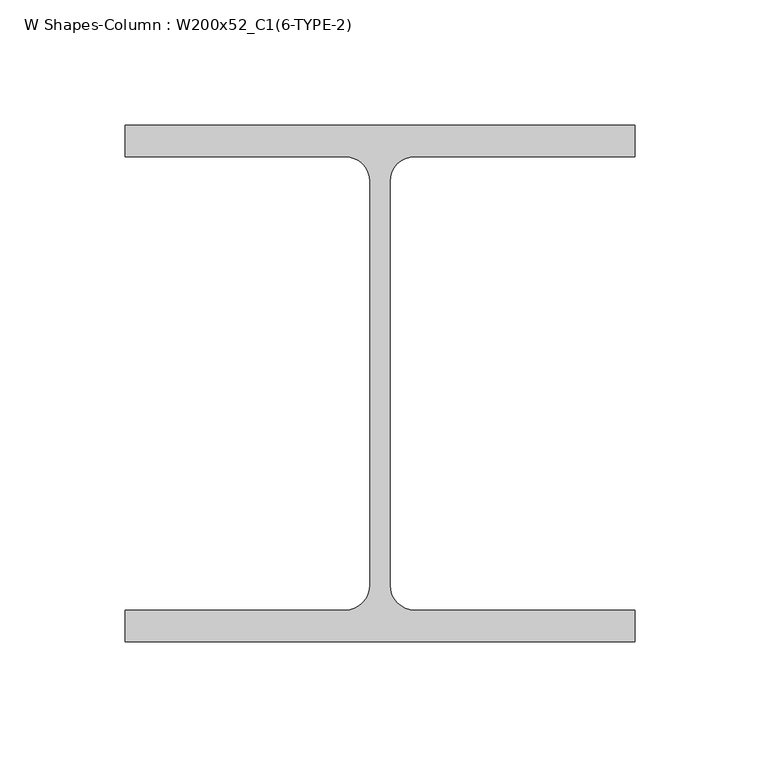
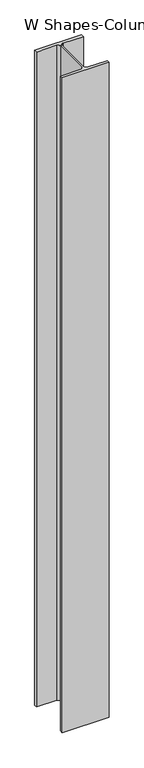
"""IFC4 building model written with IfcOpenShell, lengths in millimetres: column geometry, W Shapes-Column : W200x52_C1(6-TYPE-2)."""

from ifc_helpers import new_model, si_unit, point, frame, frame_2d, origin, place, context, project, spatial, polyline, circle_curve, trimmed, segment, composite_curve, outline, extrude, source, transform, mapped, element, save


def w_shapes_column_w200x52_c1_6_type_2_a0398fbe(model_context):
    return source(origin(), model_context, "Body", "SweptSolid", [
        extrude(outline(composite_curve([segment(polyline([(101.854, -103.124), (-101.854, -103.124), (-101.854, -90.551), (-13.9446, -90.551)]), True, "CONTINUOUS"), segment(trimmed(circle_curve(frame_2d((-13.9446, -80.5434)), 10.0076), [point((-13.9446, -90.551))], [point((-3.937, -80.5434))], True, "CARTESIAN"), True, "CONTINUOUS"), segment(polyline([(-3.937, -80.5434), (-3.937, 80.5434)]), True, "CONTINUOUS"), segment(trimmed(circle_curve(frame_2d((-13.9446, 80.5434)), 10.0076), [point((-3.937, 80.5434))], [point((-13.9446, 90.551))], True, "CARTESIAN"), True, "CONTINUOUS"), segment(polyline([(-13.9446, 90.551), (-101.854, 90.551), (-101.854, 103.124), (101.854, 103.124), (101.854, 90.551), (13.9446, 90.551)]), True, "CONTINUOUS"), segment(trimmed(circle_curve(frame_2d((13.9446, 80.5434)), 10.0076), [point((13.9446, 90.551))], [point((3.937, 80.5434))], True, "CARTESIAN"), True, "CONTINUOUS"), segment(polyline([(3.937, 80.5434), (3.937, -80.5434)]), True, "CONTINUOUS"), segment(trimmed(circle_curve(frame_2d((13.9446, -80.5434)), 10.0076), [point((3.937, -80.5434))], [point((13.9446, -90.551))], True, "CARTESIAN"), True, "CONTINUOUS"), segment(polyline([(13.9446, -90.551), (101.854, -90.551), (101.854, -103.124)]), True, "CONTINUOUS")], self_intersect=False)), frame((0.0, 0.0, 3220.0), z_axis=(0.0, 0.0, 1.0), x_axis=(1.0, 0.0, 0.0)), (0.0, 0.0, 1.0), 3000.0),
    ])


if __name__ == "__main__":
    model = new_model("IFC4")
    model_context = context("Model", 3, world=origin())
    ifc_project = project(units=[si_unit("LENGTHUNIT", "METRE", prefix="MILLI")], contexts=[model_context])
    site = spatial("IfcSite", under=ifc_project)
    building = spatial("IfcBuilding", under=site)
    placement = place(None, origin())
    w_shapes_column_w200x52_c1_6_type_2_shape = w_shapes_column_w200x52_c1_6_type_2_a0398fbe(model_context)
    element("IfcColumn", 1, ObjectType="W Shapes-Column : W200x52_C1(6-TYPE-2)", at=placement, inside=building, context=model_context, shape_type="MappedRepresentation", body=[
        mapped(w_shapes_column_w200x52_c1_6_type_2_shape, transform((0.0, 0.0, 0.0), x_axis=(1.0, 0.0, 0.0), y_axis=(0.0, 1.0, 0.0), z_axis=(0.0, 0.0, 1.0))),
    ])
    save(model, "model.ifc")

# Revit data of these elements
# Type "W Shapes-Column : W200x52_C1(6-TYPE-2)"
#   Section Name Key = "W8X35"
#   Assembly Code = "B10"
#   Width = 20.3708 cm
#   Web Thickness = 0.7874 cm
#   Web Fillet = 1.0008 cm
#   Warping Constant = 166223.7 cm⁶
#   Torsional Moment of Inertia = 32.0082 cm⁴
#   Section Area = 66.4515 cm²
#   Plastic Modulus weak axis = 263.832 cm³
#   Plastic Modulus strong axis = 568.631 cm³
#   Perimeter = 1.1936 m²/m
#   Nominal Weight = 52.0857 kgf/m
#   Moment of Inertia weak axis = 1773.15 cm⁴
#   Moment of Inertia strong axis = 5286.14 cm⁴
#   Height = 20.6248 cm
#   Flange Thickness = 1.2573 cm
#   Elastic Modulus weak axis = 173.703 cm³
#   Elastic Modulus strong axis = 511.276 cm³
#   Clear Web Height = 14.605 cm
#   Centroid Vertical = 10.3124 cm
#   Centroid Horizontal = 10.1854 cm
#   Bolt Spacing = 13.97 cm
#   Structural Material [instance default] = Steel ASTM A992
#   Principal Axes Angle = 0
# Element 1 (IfcColumn, "W Shapes-Column : W200x52_C1(6-TYPE-2)")
#   Structural Material = none
# Materials
#   "Steel ASTM A992": class "Metal", colour RGB 199 199 199, transparency 0, Description = "Structural steel 50ksi", Cost = 0
